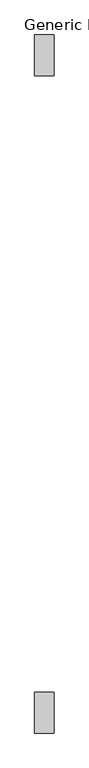
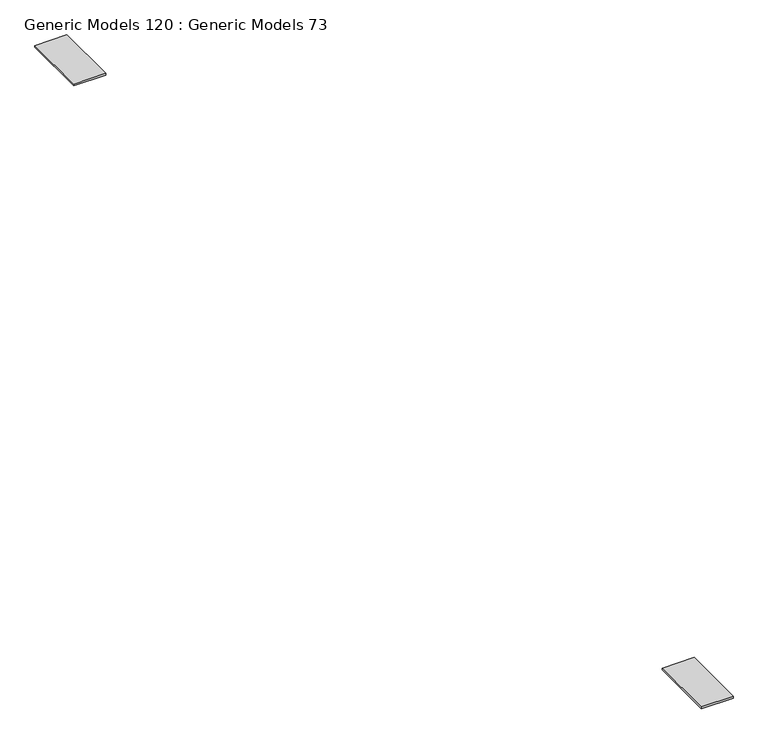
"""IFC4 building model written with IfcOpenShell, lengths in millimetres: proxy geometry, Generic Models 120 : Generic Models 73."""

from ifc_helpers import new_model, si_unit, frame, origin, place, context, project, spatial, polyline, outline, extrude, source, transform, mapped, element, save


def generic_models_120_generic_models_73_a88c3939(model_context):
    return source(origin(), model_context, "Body", "SweptSolid", [
        extrude(outline(polyline([(32040.4971032, 30964.2606313), (32040.4971032, 30690.2031612), (31910.3221032, 30690.2031612), (31910.3221032, 30964.2606313), (32040.4971032, 30964.2606313)])), frame((0.0, 0.0, 266414.25), z_axis=(0.0, 0.0, 1.0), x_axis=(1.0, 0.0, 0.0)), (0.0, 0.0, 1.0), 7.9375),
        extrude(outline(polyline([(32040.4971032, 35373.9582942), (32040.4971032, 35100.8368035), (31910.3221032, 35100.8368035), (31910.3221032, 35373.9582942), (32040.4971032, 35373.9582942)])), frame((0.0, 0.0, 266414.25), z_axis=(0.0, 0.0, 1.0), x_axis=(1.0, 0.0, 0.0)), (0.0, 0.0, 1.0), 7.9375),
    ])


if __name__ == "__main__":
    model = new_model("IFC4")
    model_context = context("Model", 3, world=origin())
    ifc_project = project(units=[si_unit("LENGTHUNIT", "METRE", prefix="MILLI")], contexts=[model_context])
    site = spatial("IfcSite", under=ifc_project)
    building = spatial("IfcBuilding", under=site)
    placement = place(None, origin())
    generic_models_120_generic_models_73_shape = generic_models_120_generic_models_73_a88c3939(model_context)
    element("IfcBuildingElementProxy", 1, Name="Generic Models 120 : Generic Models 73", ObjectType="Generic Models 120 : Generic Models 73", at=placement, inside=building, context=model_context, shape_type="MappedRepresentation", body=[
        mapped(generic_models_120_generic_models_73_shape, transform((0.0, 0.0, 0.0), x_axis=(1.0, 0.0, 0.0), y_axis=(0.0, 1.0, 0.0), z_axis=(0.0, 0.0, 1.0))),
    ])
    save(model, "model.ifc")

# Revit data of these elements
# Element 1 (IfcBuildingElementProxy, "Generic Models 120 : Generic Models 73")
#   Materials on its faces: "6 x 5/8\" BASE PL. W/ (2) \n5/8\" EMBEDMENT EPOXY ANCHORS"
# Materials
#   "6 x 5/8\" BASE PL. W/ (2) \n5/8\" EMBEDMENT EPOXY ANCHORS": class "Metal", colour RGB 199 199 199, transparency 0, Description = "Carbon steel", Cost = 0
